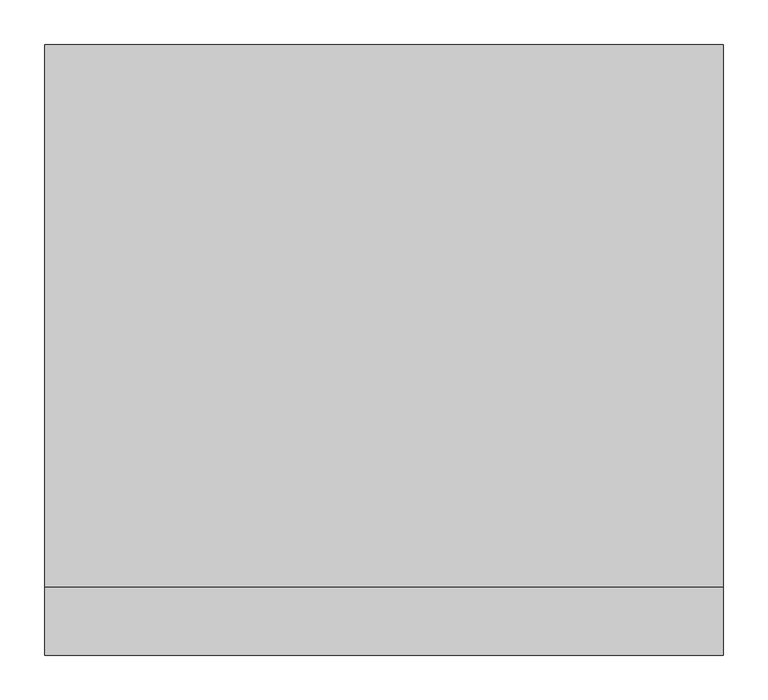
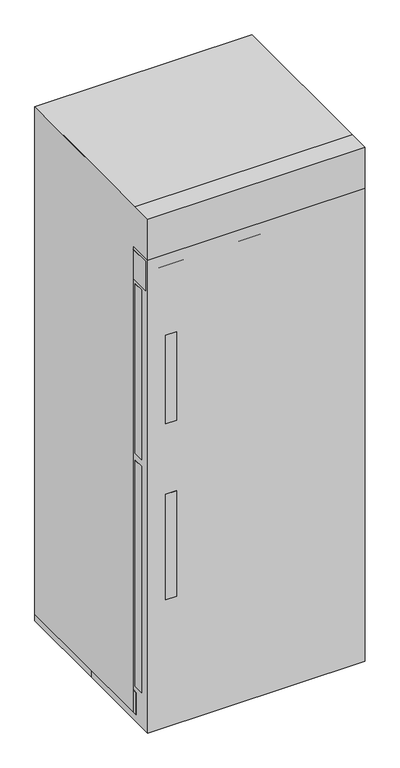
"""IFC4 building model written with IfcOpenShell, lengths in millimetres: proxy geometry, M3110 - Cabinet, Warming, F-S, 2 Heated Compartment, Elect : M3110 - Cabinet, Warming, F-S, 2 Heated Compartment, Elect."""

import ifcopenshell
import ifcopenshell.guid

model = None  # the IFC model being written
_history = None  # IfcOwnerHistory: only IFC2X3 demands one
_inside = {}  # id of a spatial element -> (the spatial element, [elements in it])
_under = {}  # id of a project, library or spatial element -> (it, [spatial elements below it])
_declared = {}  # id of a project -> (the project, [libraries it declares])
_typed = {}  # id of a type object -> (the type object, [elements of that type])
_made_of = {}  # id of a material, layer set ... -> (it, [elements and type objects made of it])


def new_model(schema):
    """Start an empty IFC model of exactly this schema.

    Asked for "IFC4X3", IfcOpenShell would pick the latest addendum, in which some entities
    have other attributes; the version numbers below select the first issue.
    IFC2X3 requires an IfcOwnerHistory on every rooted entity: one is made here for all.
    """
    global model, _history
    if schema == "IFC4X3":
        model = ifcopenshell.file(schema_version=(4, 3, 0, 0))
    else:
        model = ifcopenshell.file(schema=schema)
    _inside.clear()
    _under.clear()
    _declared.clear()
    _typed.clear()
    _made_of.clear()
    _history = None
    if model.schema == "IFC2X3":
        org = make("IfcOrganization", Name="unknown")
        user = make(
            "IfcPersonAndOrganization",
            ThePerson=make("IfcPerson", FamilyName="unknown"),
            TheOrganization=org,
        )
        app = make(
            "IfcApplication",
            ApplicationDeveloper=org,
            Version="unknown",
            ApplicationFullName="unknown",
            ApplicationIdentifier="unknown",
        )
        _history = make(
            "IfcOwnerHistory",
            OwningUser=user,
            OwningApplication=app,
            ChangeAction="ADDED",
            CreationDate=0,
        )
    return model


def make(cls, **values):
    """One entity of the class cls with the attributes given. An attribute that is None is left unset."""
    return model.create_entity(
        cls, **{name: value for name, value in values.items() if value is not None}
    )


def rooted(cls, **values):
    """An entity with a GlobalId (a new one), such as an element, a storey or a relation."""
    return make(cls, GlobalId=ifcopenshell.guid.new(), OwnerHistory=_history, **values)


def si_unit(unit_type, name, prefix=None):
    """IfcSIUnit, for example si_unit("LENGTHUNIT", "METRE", prefix="MILLI")."""
    return make("IfcSIUnit", UnitType=unit_type, Prefix=prefix, Name=name)


def assignment(units):
    """IfcUnitAssignment: the units of a project."""
    return None if units is None else make("IfcUnitAssignment", Units=units)


def point(xyz):
    """IfcCartesianPoint."""
    return None if xyz is None else make("IfcCartesianPoint", Coordinates=xyz)


def direction(xyz):
    """IfcDirection."""
    return None if xyz is None else make("IfcDirection", DirectionRatios=xyz)


def frame(location, z_axis=None, x_axis=None):
    """IfcAxis2Placement3D, a coordinate frame: its origin and axes. An axis left out is left unset."""
    return make(
        "IfcAxis2Placement3D",
        Location=point(location),
        Axis=direction(z_axis),
        RefDirection=direction(x_axis),
    )


def frame_2d(location, x_axis=None):
    """IfcAxis2Placement2D, a coordinate frame in the plane: its origin and x axis."""
    return make(
        "IfcAxis2Placement2D", Location=point(location), RefDirection=direction(x_axis)
    )


def origin():
    """The frame at (0, 0, 0) with its axes left unset."""
    return frame((0.0, 0.0, 0.0))


def origin_with_axes():
    """The frame at (0, 0, 0) with the z axis (0, 0, 1) and the x axis (1, 0, 0) written out."""
    return frame((0.0, 0.0, 0.0), z_axis=(0.0, 0.0, 1.0), x_axis=(1.0, 0.0, 0.0))


def place(relative_to, where):
    """IfcLocalPlacement: puts the frame where relative to a parent placement (None: the world)."""
    return make(
        "IfcLocalPlacement", PlacementRelTo=relative_to, RelativePlacement=where
    )


def context(
    kind, dimensions, precision=None, world=None, true_north=None, identifier=None
):
    """IfcGeometricRepresentationContext, for example the 3D "Model" context."""
    return make(
        "IfcGeometricRepresentationContext",
        ContextIdentifier=identifier,
        ContextType=kind,
        CoordinateSpaceDimension=dimensions,
        Precision=precision,
        WorldCoordinateSystem=world,
        TrueNorth=true_north,
    )


def project(units=None, contexts=None):
    """IfcProject with its units and contexts."""
    return rooted(
        "IfcProject",
        Name="project",
        RepresentationContexts=contexts,
        UnitsInContext=assignment(units),
    )


def spatial(cls, under=None, at=None, **own):
    """A site, building, storey or space (cls), placed at a placement, below another one or the project."""
    s = rooted(cls, ObjectPlacement=at, **own)
    if under is not None:
        _under.setdefault(under.id(), (under, []))[1].append(s)
    return s


def polyline(points):
    """IfcPolyline through the points."""
    return make("IfcPolyline", Points=[point(p) for p in points])


def circle_curve(where, radius):
    """IfcCircle in the frame where."""
    return make("IfcCircle", Position=where, Radius=radius)


def trimmed(basis, trim1, trim2, sense, master):
    """IfcTrimmedCurve: the piece of a basis curve between two trims."""
    return make(
        "IfcTrimmedCurve",
        BasisCurve=basis,
        Trim1=trim1,
        Trim2=trim2,
        SenseAgreement=sense,
        MasterRepresentation=master,
    )


def segment(curve, same_sense, transition):
    """IfcCompositeCurveSegment."""
    return make(
        "IfcCompositeCurveSegment",
        Transition=transition,
        SameSense=same_sense,
        ParentCurve=curve,
    )


def composite_curve(segments, self_intersect=None):
    """IfcCompositeCurve: segments joined end to end."""
    return make("IfcCompositeCurve", Segments=segments, SelfIntersect=self_intersect)


def outline(outer, holes=None, kind="AREA"):
    """IfcArbitraryClosedProfileDef: a profile drawn as a closed curve; with holes, ...WithVoids."""
    if holes is None:
        return make("IfcArbitraryClosedProfileDef", ProfileType=kind, OuterCurve=outer)
    return make(
        "IfcArbitraryProfileDefWithVoids",
        ProfileType=kind,
        OuterCurve=outer,
        InnerCurves=holes,
    )


def extrude(swept, where, along, depth):
    """IfcExtrudedAreaSolid: the profile swept, set in the frame where, extruded along a direction by depth."""
    return make(
        "IfcExtrudedAreaSolid",
        SweptArea=swept,
        Position=where,
        ExtrudedDirection=direction(along),
        Depth=depth,
    )


def shape(context_of_items, identifier, shape_type, items):
    """IfcShapeRepresentation: the items that make up one representation, for example the "Body"."""
    return make(
        "IfcShapeRepresentation",
        ContextOfItems=context_of_items,
        RepresentationIdentifier=identifier,
        RepresentationType=shape_type,
        Items=items,
    )


def source(mapping_origin, context_of_items, identifier, shape_type, items):
    """IfcRepresentationMap: a shape defined once, which mapped items show again and again."""
    return make(
        "IfcRepresentationMap",
        MappingOrigin=mapping_origin,
        MappedRepresentation=shape(context_of_items, identifier, shape_type, items),
    )


def transform(
    local_origin,
    x_axis=None,
    y_axis=None,
    z_axis=None,
    scale=None,
    scale2=None,
    scale3=None,
    uniform=True,
):
    """IfcCartesianTransformationOperator3D, or its non-uniform kind. x_axis, y_axis, z_axis: its Axis1, 2, 3."""
    if uniform:
        return make(
            "IfcCartesianTransformationOperator3D",
            Axis1=direction(x_axis),
            Axis2=direction(y_axis),
            LocalOrigin=point(local_origin),
            Scale=scale,
            Axis3=direction(z_axis),
        )
    return make(
        "IfcCartesianTransformationOperator3DnonUniform",
        Axis1=direction(x_axis),
        Axis2=direction(y_axis),
        LocalOrigin=point(local_origin),
        Scale=scale,
        Axis3=direction(z_axis),
        Scale2=scale2,
        Scale3=scale3,
    )


def mapped(mapping_source, mapping_target):
    """IfcMappedItem: shows the shape of a source again, moved by a transform."""
    return make(
        "IfcMappedItem", MappingSource=mapping_source, MappingTarget=mapping_target
    )


def made_of(thing, what):
    """Note that an element or type object is made of a material, layer set ...; save() writes the relation."""
    if what is not None:
        _made_of.setdefault(what.id(), (what, []))[1].append(thing)
    return thing


def element(
    cls,
    number,
    at=None,
    inside=None,
    cuts=None,
    type_object=None,
    material=None,
    context=None,
    identifier="Body",
    shape_type=None,
    held_by="IfcProductDefinitionShape",
    body=None,
    shapes=None,
    **own,
):
    """One element of the class cls, such as IfcWall. Its Tag is "e" and its number.

    at: its placement. inside: the storey or other place that contains it. cuts: it is an
    opening in that element (IfcRelVoidsElement). A single representation is given by context,
    identifier, shape_type and body (its items); several are given by shapes. held_by: the class
    of the entity that holds the representations. save() writes the other relations.
    """
    e = rooted(cls, Tag="e%d" % number, ObjectPlacement=at, **own)
    if body is not None:
        shapes = [shape(context, identifier, shape_type, body)]
    if shapes is not None:
        e.Representation = make(held_by, Representations=shapes)
    if inside is not None:
        _inside.setdefault(inside.id(), (inside, []))[1].append(e)
    if cuts is not None:
        rooted(
            "IfcRelVoidsElement", RelatingBuildingElement=cuts, RelatedOpeningElement=e
        )
    if type_object is not None:
        _typed.setdefault(type_object.id(), (type_object, []))[1].append(e)
    return made_of(e, material)


def aggregate(whole, parts):
    """IfcRelAggregates: a whole, such as a stair, and the parts it consists of."""
    return rooted("IfcRelAggregates", RelatingObject=whole, RelatedObjects=parts)


def save(model, path):
    """Write the relations noted so far, then the file.

    IfcRelAggregates (storeys below a building ...), IfcRelContainedInSpatialStructure (elements
    in a storey), IfcRelDefinesByType, IfcRelAssociatesMaterial and IfcRelDeclares: one each for
    every whole, place, type object, material and project.
    """
    for whole, parts in _under.values():
        aggregate(whole, parts)
    for where, things in _inside.values():
        rooted(
            "IfcRelContainedInSpatialStructure",
            RelatedElements=things,
            RelatingStructure=where,
        )
    for kind, things in _typed.values():
        rooted("IfcRelDefinesByType", RelatedObjects=things, RelatingType=kind)
    for what, things in _made_of.values():
        rooted("IfcRelAssociatesMaterial", RelatedObjects=things, RelatingMaterial=what)
    for by, libraries in _declared.values():
        rooted("IfcRelDeclares", RelatingContext=by, RelatedDefinitions=libraries)
    model.write(path)


def specialty_equipment_4f3136f0(model_context):
    return source(origin(), model_context, "Body", "SweptSolid", [
        extrude(outline(polyline([(-219.4498767, -341.8038063), (-340.0998767, -341.8038063), (-340.0998767, -329.1038063), (-219.4498767, -329.1038063), (-219.4498767, -341.8038063)])), frame((0.0, 0.0, 1672.5086108), z_axis=(0.0, 0.0, 1.0), x_axis=(1.0, 0.0, 0.0)), (0.0, 0.0, 1.0), 38.1),
        extrude(outline(polyline([(60.325, -341.8038063), (-60.325, -341.8038063), (-60.325, -329.1038063), (60.325, -329.1038063), (60.325, -341.8038063)])), frame((0.0, 0.0, 1672.5086108), z_axis=(0.0, 0.0, 1.0), x_axis=(1.0, 0.0, 0.0)), (0.0, 0.0, 1.0), 38.1),
        extrude(outline(polyline([(340.0998767, -341.8038063), (219.4498767, -341.8038063), (219.4498767, -329.1038063), (340.0998767, -329.1038063), (340.0998767, -341.8038063)])), frame((0.0, 0.0, 1672.5086108), z_axis=(0.0, 0.0, 1.0), x_axis=(1.0, 0.0, 0.0)), (0.0, 0.0, 1.0), 38.1),
        extrude(outline(polyline([(-266.7, 1905.0), (342.9, 1905.0), (342.9, 25.4), (-254.0, 25.4), (-254.0, 1752.6), (-342.9, 1752.6), (-342.9, 1905.0), (-266.7, 1905.0)])), frame((-381.0, 0.0, 0.0), z_axis=(1.0, 0.0, 0.0), x_axis=(0.0, 1.0, 0.0)), (0.0, 0.0, 1.0), 762.0),
        extrude(outline(polyline([(381.0, -254.0), (381.0, -329.1038063), (-381.0, -329.1038063), (-381.0, -254.0), (381.0, -254.0)])), frame((0.0, 0.0, 1631.95), z_axis=(0.0, 0.0, 1.0), x_axis=(1.0, 0.0, 0.0)), (0.0, 0.0, 1.0), 107.95),
        extrude(outline(polyline([(-342.9, 1451.7534297), (-304.8, 1451.7534297), (-304.8, 1439.0534297), (-330.2159299, 1439.0534297), (-330.2159299, 1136.6340701), (-304.8, 1136.6340701), (-304.8, 1123.95), (-342.9, 1123.95), (-342.9, 1451.7534297)])), frame((-317.5, 0.0, 0.0), z_axis=(1.0, 0.0, 0.0), x_axis=(0.0, 1.0, 0.0)), (0.0, 0.0, 1.0), 38.1),
        extrude(outline(polyline([(-342.9, 471.6629987), (-342.9, 863.1515947), (-304.8, 863.1515947), (-304.8, 850.4675247), (-330.2159299, 850.4675247), (-330.2159299, 484.3629987), (-304.8, 484.3629987), (-304.8, 471.6629987), (-342.9, 471.6629987)])), frame((-317.5, 0.0, 0.0), z_axis=(1.0, 0.0, 0.0), x_axis=(0.0, 1.0, 0.0)), (0.0, 0.0, 1.0), 38.1),
        extrude(outline(polyline([(381.0, -254.0), (381.0, -273.05), (-381.0, -273.05), (-381.0, -254.0), (381.0, -254.0)])), frame((0.0, 0.0, 25.4), z_axis=(0.0, 0.0, 1.0), x_axis=(1.0, 0.0, 0.0)), (0.0, 0.0, 1.0), 82.55),
        extrude(outline(polyline([(368.3, -266.7), (-368.3, -266.7), (-368.3, -254.0), (368.3, -254.0), (368.3, -266.7)])), frame((0.0, 0.0, 1006.24443), z_axis=(0.0, 0.0, 1.0), x_axis=(1.0, 0.0, 0.0)), (0.0, 0.0, 1.0), 587.60557),
        extrude(outline(polyline([(381.0, -304.8), (-381.0, -304.8), (-381.0, -266.7), (381.0, -266.7), (381.0, -304.8)])), frame((0.0, 0.0, 990.6), z_axis=(0.0, 0.0, 1.0), x_axis=(1.0, 0.0, 0.0)), (0.0, 0.0, 1.0), 628.65),
        extrude(outline(polyline([(368.3, -266.7), (-368.3, -266.7), (-368.3, -254.0), (368.3, -254.0), (368.3, -266.7)])), frame((0.0, 0.0, 149.0357475), z_axis=(0.0, 0.0, 1.0), x_axis=(1.0, 0.0, 0.0)), (0.0, 0.0, 1.0), 797.1142525),
        extrude(outline(polyline([(381.0, -304.8), (-381.0, -304.8), (-381.0, -266.7), (381.0, -266.7), (381.0, -304.8)])), frame((0.0, 0.0, 126.9407444), z_axis=(0.0, 0.0, 1.0), x_axis=(1.0, 0.0, 0.0)), (0.0, 0.0, 1.0), 838.2592556),
        extrude(outline(composite_curve([segment(trimmed(circle_curve(frame_2d((-307.8775617, -192.5820241)), 31.75), [point((-276.1275617, -192.5820241))], [point((-339.6275617, -192.5820241))], False, "CARTESIAN"), True, "CONTINUOUS"), segment(trimmed(circle_curve(frame_2d((-307.8775617, -192.5820241)), 31.75), [point((-339.6275617, -192.5820241))], [point((-276.1275617, -192.5820241))], False, "CARTESIAN"), True, "CONTINUOUS")], self_intersect=False)), origin_with_axes(), (0.0, 0.0, 1.0), 25.4),
        extrude(outline(composite_curve([segment(trimmed(circle_curve(frame_2d((307.8775617, -192.5820241)), 31.75), [point((276.1275617, -192.5820241))], [point((339.6275617, -192.5820241))], False, "CARTESIAN"), True, "CONTINUOUS"), segment(trimmed(circle_curve(frame_2d((307.8775617, -192.5820241)), 31.75), [point((339.6275617, -192.5820241))], [point((276.1275617, -192.5820241))], False, "CARTESIAN"), True, "CONTINUOUS")], self_intersect=False)), origin_with_axes(), (0.0, 0.0, 1.0), 25.4),
        extrude(outline(composite_curve([segment(trimmed(circle_curve(frame_2d((-307.8775617, 277.3179759)), 31.75), [point((-276.1275617, 277.3179759))], [point((-339.6275617, 277.3179759))], False, "CARTESIAN"), True, "CONTINUOUS"), segment(trimmed(circle_curve(frame_2d((-307.8775617, 277.3179759)), 31.75), [point((-339.6275617, 277.3179759))], [point((-276.1275617, 277.3179759))], False, "CARTESIAN"), True, "CONTINUOUS")], self_intersect=False)), origin_with_axes(), (0.0, 0.0, 1.0), 25.4),
        extrude(outline(composite_curve([segment(trimmed(circle_curve(frame_2d((307.8775617, 277.3179759)), 31.75), [point((276.1275617, 277.3179759))], [point((339.6275617, 277.3179759))], False, "CARTESIAN"), True, "CONTINUOUS"), segment(trimmed(circle_curve(frame_2d((307.8775617, 277.3179759)), 31.75), [point((339.6275617, 277.3179759))], [point((276.1275617, 277.3179759))], False, "CARTESIAN"), True, "CONTINUOUS")], self_intersect=False)), origin_with_axes(), (0.0, 0.0, 1.0), 25.4),
        extrude(outline(polyline([(-381.0, 342.9), (381.0, 342.9), (381.0, -342.9), (-381.0, -342.9), (-381.0, 0.0), (-381.0, 342.9)])), origin_with_axes(), (0.0, 0.0, 1.0), 1905.0),
    ])


if __name__ == "__main__":
    model = new_model("IFC4")
    model_context = context("Model", 3, world=origin())
    ifc_project = project(units=[si_unit("LENGTHUNIT", "METRE", prefix="MILLI")], contexts=[model_context])
    site = spatial("IfcSite", under=ifc_project)
    building = spatial("IfcBuilding", under=site)
    placement = place(None, origin())
    specialty_equipment_shape = specialty_equipment_4f3136f0(model_context)
    element("IfcBuildingElementProxy", 1, Name="M3110 - Cabinet, Warming, F-S, 2 Heated Compartment, Elect : M3110 - Cabinet, Warming, F-S, 2 Heated Compartment, Elect", ObjectType="M3110 - Cabinet, Warming, F-S, 2 Heated Compartment, Elect : M3110 - Cabinet, Warming, F-S, 2 Heated Compartment, Elect", at=placement, inside=building, context=model_context, shape_type="MappedRepresentation", body=[
        mapped(specialty_equipment_shape, transform((0.0, 0.0, 0.0), x_axis=(1.0, 0.0, 0.0), y_axis=(0.0, 1.0, 0.0), z_axis=(0.0, 0.0, 1.0))),
    ])
    save(model, "model.ifc")

# Revit data of these elements
# Project information
#   Room Abbreviation = "RRSS1"
#   Room Description = "Recovery Station, Phase I (RRSS1)"
#   Sheets - Total = "5"
#   Project Issue Date = "Issue Date"
#   Project Status = "Project Status"
#   Client Name = "Owner"
#   Project Address = "Enter address here"
#   Project Name = "Project Name"
#   Project Number = "Project Number"
#   Publication Date = "30-Jan-15"
# Type "M3110 - Cabinet, Warming, F-S, 2 Heated Compartment, Elect : M3110 - Cabinet, Warming, F-S, 2 Heated Compartment, Elect"
#   Watts2 = "0"
#   Watts1 = "1800"
#   Unit_Issue = "EA"
#   UTIL_6_Misc = "-"
#   UTIL_5_NonMedGas = "-"
#   UTIL_4_MiscGas = "-"
#   UTIL_3_MedGas = "-"
#   UTIL_2_Elec = "f"
#   UTIL_1_WaterDrain = "-"
#   Nomenclature = "Cabinet, Warming, F/S, 2 Heated Compartment, Elect"
#   NSN = "6530"
#   Location [instance default] = ""
#   JSN = "M3110"
#   Fund_Source_VA = "-"
#   Fund_Source_Navy = "-"
#   Fund_Source_Army = "-"
#   Fund_Source_AF = "-"
#   ELEC_Volts2 = "0"
#   ELEC_Volts1 = "120"
#   ELEC_Phase2 = "0"
#   ELEC_Phase1 = "1"
#   ELEC_HertzSwitch = "-1"
#   ELEC_HertzDependent = "0"
#   ELEC_Hertz = "60"
#   ELEC_Amps2 = "0"
#   ELEC_Amps1 = "15"
#   DetailDescription = "Freestanding, single or double door warming cabinet with 2 heated compartments. Compartment and exterior walls are made from stainless steel. Thick fiberglass insulation maintains the interior temperature and keeps the exterior from becoming too hot. Equipped with a sealing door, thermostatic temperature control, status display, heat indicating light, over temperature protection, alarms and an air circulating fan. Unit may have an optional temperature recorder. Manufacturer recommends using a fused disconnect switch in the electrical power circuit. Cabinet may also be installed in a recess. Designed for heating and storing solutions and blankets used in patient care areas."
#   CAT_VA = "A"
#   CAT_Navy = "A"
#   CAT_IHS = "-"
#   CAT_Army = "A"
#   CAT_AF = "A"
#   BTUperhour = "0"
#   Weight_IP = 498
#   DIM_Width_IP = 2' - 6"
#   DIM_Height_IP = 6' - 3"
#   DIM_Depth_IP = 2' - 3"
# Element 1 (IfcBuildingElementProxy, "M3110 - Cabinet, Warming, F-S, 2 Heated Compartment, Elect : M3110 - Cabinet, Warming, F-S, 2 Heated Compartment, Elect")
#   Location = "RRSS1"
